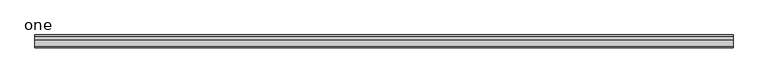
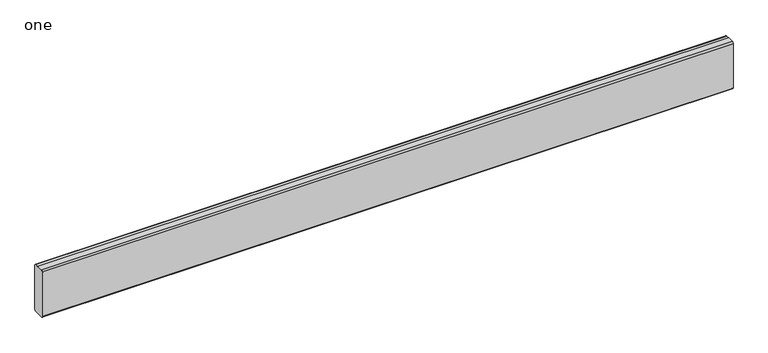
"""IFC4 building model written with IfcOpenShell, lengths in millimetres: beam geometry, Trex : one."""

from ifc_helpers import new_model, si_unit, point, frame, frame_2d, origin, place, context, project, spatial, polyline, circle_curve, trimmed, segment, composite_curve, outline, extrude, source, transform, mapped, element, save


def one_c02e0670(model_context):
    return source(origin(), model_context, "Body", "SweptSolid", [
        extrude(outline(composite_curve([segment(polyline([(4.9179935, -103.2371094), (-19.7941406, -103.2371094)]), True, "CONTINUOUS"), segment(trimmed(circle_curve(frame_2d((-19.7941406, -96.8871094)), 6.35), [point((-19.7941406, -103.2371094))], [point((-26.1441406, -96.8871094))], False, "CARTESIAN"), True, "CONTINUOUS"), segment(polyline([(-26.1441406, -96.8871094), (-26.1441406, 96.8871094)]), True, "CONTINUOUS"), segment(trimmed(circle_curve(frame_2d((-19.7941406, 96.8871094)), 6.35), [point((-26.1441406, 96.8871094))], [point((-19.7941406, 103.2371094))], False, "CARTESIAN"), True, "CONTINUOUS"), segment(polyline([(-19.7941406, 103.2371094), (4.9179935, 103.2371094), (4.9179935, 101.6496094), (19.7941406, 101.6496094)]), True, "CONTINUOUS"), segment(trimmed(circle_curve(frame_2d((19.7941406, 95.2996094)), 6.35), [point((19.7941406, 101.6496094))], [point((26.1441406, 95.2996094))], False, "CARTESIAN"), True, "CONTINUOUS"), segment(polyline([(26.1441406, 95.2996094), (26.1441406, -95.2996094)]), True, "CONTINUOUS"), segment(trimmed(circle_curve(frame_2d((19.7941406, -95.2996094)), 6.35), [point((26.1441406, -95.2996094))], [point((19.7941406, -101.6496094))], False, "CARTESIAN"), True, "CONTINUOUS"), segment(polyline([(19.7941406, -101.6496094), (4.9179935, -101.6496094), (4.9179935, -103.2371094)]), True, "CONTINUOUS")], self_intersect=False)), frame((-1470.7697009, 0.0, 0.0), z_axis=(1.0, 0.0, 0.0), x_axis=(0.0, 1.0, 0.0)), (0.0, 0.0, 1.0), 2853.0942979),
    ])


if __name__ == "__main__":
    model = new_model("IFC4")
    model_context = context("Model", 3, world=origin())
    ifc_project = project(units=[si_unit("LENGTHUNIT", "METRE", prefix="MILLI")], contexts=[model_context])
    site = spatial("IfcSite", under=ifc_project)
    building = spatial("IfcBuilding", under=site)
    placement = place(None, origin())
    one_shape = one_c02e0670(model_context)
    element("IfcBeam", 1, ObjectType="Trex : one", at=placement, inside=building, context=model_context, shape_type="MappedRepresentation", body=[
        mapped(one_shape, transform((0.0, 0.0, 0.0), x_axis=(1.0, 0.0, 0.0), y_axis=(0.0, 1.0, 0.0), z_axis=(0.0, 0.0, 1.0))),
    ])
    save(model, "model.ifc")

# Revit data of these elements
# Type "Trex : one"
#   Width = 0' - 2 15/256"
#   Web_Thickness = 0' - 0 7/64"
#   Length [instance default] = 10' - 0"
#   Leg_1 = 0' - 2 1/2"
#   Height = 0' - 8 33/256"
#   Structural Material [instance default] = none
